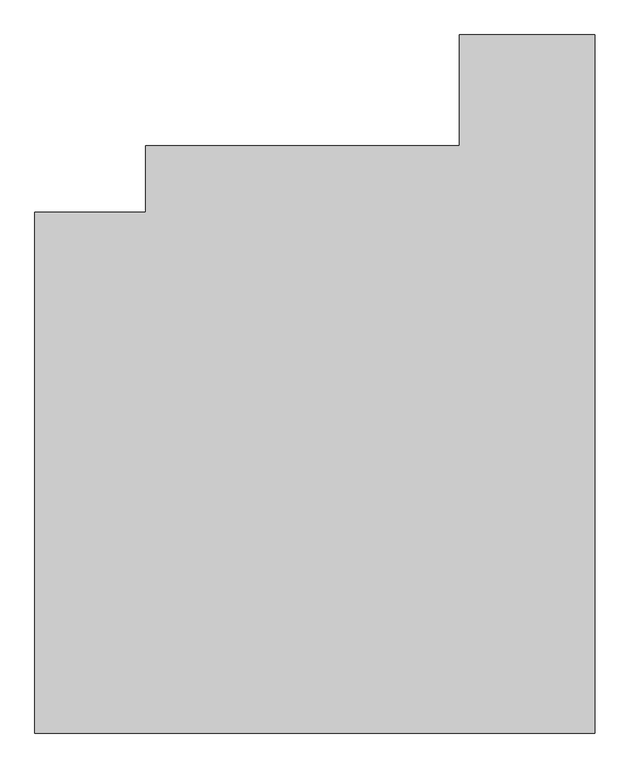
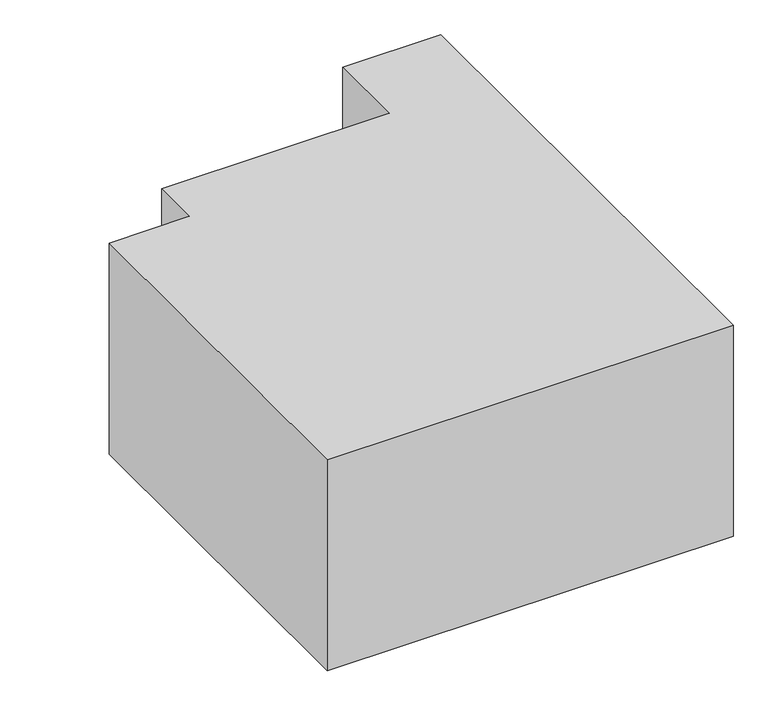
"""IFC4 building model written with IfcOpenShell, lengths in millimetres: proxy geometry, 0_3d_modell."""

from ifc_helpers import new_model, si_unit, origin, origin_with_axes, place, context, project, spatial, polyline, outline, extrude, source, transform, mapped, element, save


def generic_models_72ab0ecd(model_context):
    return source(origin(), model_context, "Body", "SweptSolid", [
        extrude(outline(polyline([(0.0, 0.2079549), (0.0, 4230.0), (900.0, 4230.0), (900.0, 4770.0), (3450.0, 4770.0), (3450.0, 5670.0), (4550.0, 5670.0), (4550.0, 0.0), (0.0, 0.2079549)])), origin_with_axes(), (0.0, 0.0, 1.0), 2500.0),
    ])


if __name__ == "__main__":
    model = new_model("IFC4")
    model_context = context("Model", 3, world=origin())
    ifc_project = project(units=[si_unit("LENGTHUNIT", "METRE", prefix="MILLI")], contexts=[model_context])
    site = spatial("IfcSite", under=ifc_project)
    building = spatial("IfcBuilding", under=site)
    placement = place(None, origin())
    generic_models_shape = generic_models_72ab0ecd(model_context)
    element("IfcBuildingElementProxy", 1, Name="0_3d_modell", ObjectType="0_3d_modell", at=placement, inside=building, context=model_context, shape_type="MappedRepresentation", body=[
        mapped(generic_models_shape, transform((0.0, 0.0, 0.0), x_axis=(1.0, 0.0, 0.0), y_axis=(0.0, 1.0, 0.0), z_axis=(0.0, 0.0, 1.0))),
    ])
    save(model, "model.ifc")

# Revit data of these elements
# Element 1 (IfcBuildingElementProxy, "0_3d_modell")
#   Materials on its faces: "*1"
# Materials
#   "*1": class "Unassigned", colour RGB 175 175 175, transparency 0
